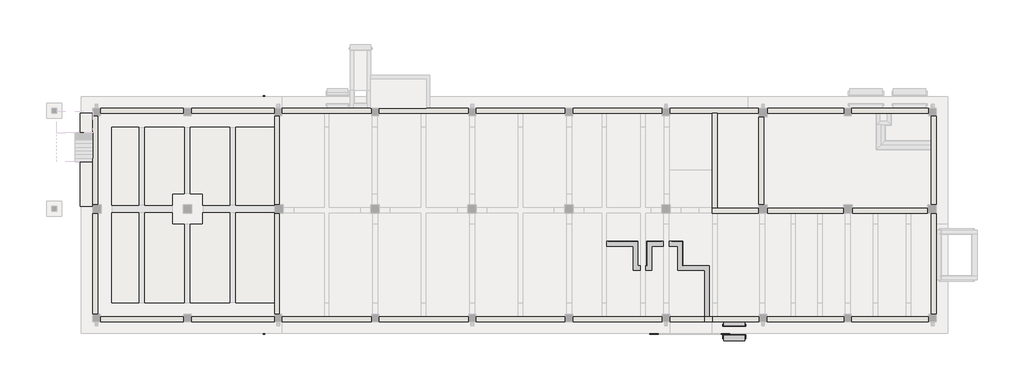
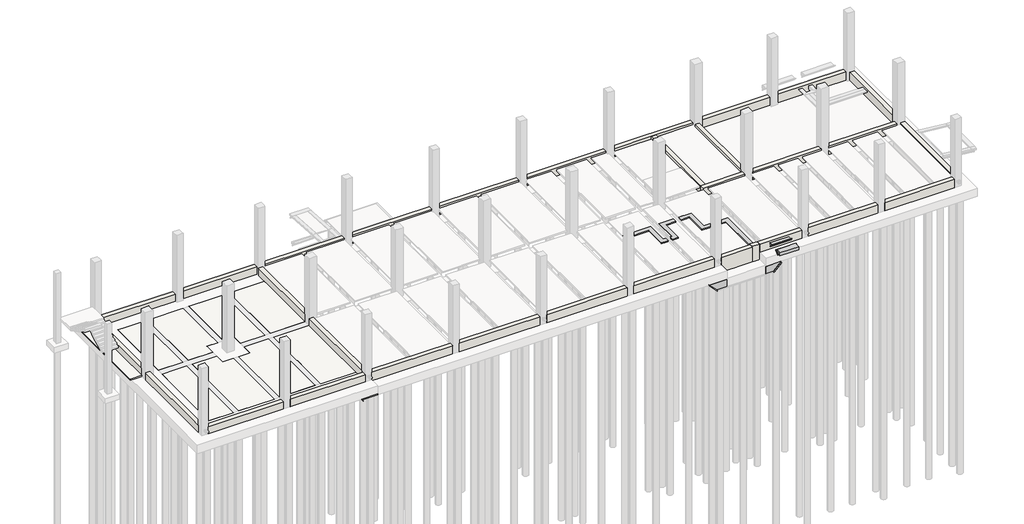
# One storey, part 1 of 7: 31 walls, 12 proxies, 4 slabs.
"""IFC4 building model written with IfcOpenShell, lengths in millimetres."""

from ifc_helpers import new_model, si_unit, frame, origin, place, context, project, spatial, polyline, outline, extrude, faceted_brep, element, save

model = new_model("IFC4")

# Units and contexts
model_context = context("Model", 3, world=origin())
ifc_project = project(units=[si_unit("LENGTHUNIT", "METRE", prefix="MILLI")], contexts=[model_context])

# Site, building, storey
site = spatial("IfcSite", under=ifc_project)
building = spatial("IfcBuilding", under=site)
storey = spatial("IfcBuildingStorey", under=building, Name="H.P.P", Elevation=4500.0)

# Proxies
placement = place(None, origin())
element("IfcBuildingElementProxy", 1, Name="H_SF_AR_S17_SOG Edge_1625x700", ObjectType="H_SF_AR_S17_SOG Edge_1625x700", at=placement, inside=storey, context=model_context, shape_type="SweptSolid", body=[
    extrude(outline(polyline([(2500.0, 47300.0), (3200.0, 47300.0), (3200.0, 45675.0), (2500.0, 46375.0), (2500.0, 47300.0)])), frame((0.0, -18250.0000001, 0.0), z_axis=(0.0, 1.0, 0.0), x_axis=(0.0, 0.0, 1.0)), (0.0, 0.0, 1.0), 2500.0),
])
element("IfcBuildingElementProxy", 2, Name="H_SF_AR_S17_SOG Edge_1400x700", ObjectType="H_SF_AR_S17_SOG Edge_1400x700", at=placement, inside=storey, context=model_context, shape_type="SweptSolid", body=[
    extrude(outline(polyline([(2500.0, 50825.0), (2500.0, 51525.0), (3200.0, 52225.0), (3200.0, 50825.0), (2500.0, 50825.0)])), frame((0.0, -18250.0000001, 0.0), z_axis=(0.0, 1.0, 0.0), x_axis=(0.0, 0.0, 1.0)), (0.0, 0.0, 1.0), 2500.0),
])
element("IfcBuildingElementProxy", 3, Name="H_SF_AR_S17_SOG Edge_1500x100", ObjectType="H_SF_AR_S17_SOG Edge_1500x100", at=placement, inside=storey, context=model_context, shape_type="SweptSolid", body=[
    extrude(outline(polyline([(3200.0, 15299.9999999), (3300.0, 15299.9999999), (3300.0, 13799.9999999), (3200.0, 13899.9999999), (3200.0, 15299.9999999)])), frame((0.0, -18250.0000001, 0.0), z_axis=(0.0, 1.0, 0.0), x_axis=(0.0, 0.0, 1.0)), (0.0, 0.0, 1.0), 2500.0),
    extrude(outline(polyline([(3200.0, 15299.9999999), (3300.0, 15299.9999999), (3300.0, 13799.9999999), (3200.0, 13899.9999999), (3200.0, 15299.9999999)])), frame((0.0, -1250.0000001, 0.0), z_axis=(0.0, 1.0, 0.0), x_axis=(0.0, 0.0, 1.0)), (0.0, 0.0, 1.0), 2500.0),
])
element("IfcBuildingElementProxy", 4, Name="H_SF_AR_S18_Lean_T50", ObjectType="H_SF_AR_S18_Lean_T50", at=placement, inside=storey, context=model_context, shape_type="SweptSolid", body=[
    extrude(outline(polyline([(3200.0, 52225.0), (2500.0, 51525.0), (2450.0, 51525.0), (2450.0, 51545.7106781), (3150.0, 52245.7106781), (3150.0, 52225.0), (3200.0, 52225.0)])), frame((0.0, -18350.0000001, 0.0), z_axis=(0.0, 1.0, 0.0), x_axis=(0.0, 0.0, 1.0)), (0.0, 0.0, 1.0), 2700.0),
])
element("IfcBuildingElementProxy", 5, Name="H_SF_AR_S18_Lean_T50", ObjectType="H_SF_AR_S18_Lean_T50", at=placement, inside=storey, context=model_context, shape_type="SweptSolid", body=[
    extrude(outline(polyline([(3200.0, 45675.0), (3150.0, 45675.0), (3150.0, 45654.2893219), (2450.0, 46354.2893219), (2450.0, 46375.0), (2500.0, 46375.0), (3200.0, 45675.0)])), frame((0.0, -18350.0000001, 0.0), z_axis=(0.0, 1.0, 0.0), x_axis=(0.0, 0.0, 1.0)), (0.0, 0.0, 1.0), 2700.0),
])
element("IfcBuildingElementProxy", 6, Name="H_SF_AR_S18_Lean_T50_100X100", ObjectType="H_SF_AR_S18_Lean_T50_100X100", at=placement, inside=storey, context=model_context, shape_type="SweptSolid", body=[
    extrude(outline(polyline([(3300.0, 13799.9999999), (3250.0, 13799.9999999), (3250.0, 13779.2893218), (3150.0, 13879.2893218), (3150.0, 13899.9999999), (3200.0, 13899.9999999), (3300.0, 13799.9999999)])), frame((0.0, -18350.0000001, 0.0), z_axis=(0.0, 1.0, 0.0), x_axis=(0.0, 0.0, 1.0)), (0.0, 0.0, 1.0), 2810.0),
    extrude(outline(polyline([(3300.0, 13799.9999999), (3250.0, 13799.9999999), (3250.0, 13779.2893218), (3150.0, 13879.2893218), (3150.0, 13899.9999999), (3200.0, 13899.9999999), (3300.0, 13799.9999999)])), frame((0.0, -1460.0000001, 0.0), z_axis=(0.0, 1.0, 0.0), x_axis=(0.0, 0.0, 1.0)), (0.0, 0.0, 1.0), 2810.0),
])
element("IfcBuildingElementProxy", 7, Name="H_SF_AR_B08_Stoop_T150_FrontEdge", ObjectType="H_SF_AR_B08_Stoop_T150_FrontEdge", at=placement, inside=storey, context=model_context, shape_type="SweptSolid", body=[
    extrude(outline(polyline([(-17312.0, 4450.0), (-17512.0, 4450.0), (-17662.0, 4600.0), (-17312.0, 4600.0), (-17312.0, 4450.0)])), frame((51775.0, 0.0, 0.0), z_axis=(1.0, 0.0, 0.0), x_axis=(0.0, 1.0, 0.0)), (0.0, 0.0, 1.0), 1700.0),
])
element("IfcBuildingElementProxy", 8, Name="H_SF_AR_B08_Stoop_T150_FrontEdge_500x300", ObjectType="H_SF_AR_B08_Stoop_T150_FrontEdge_500x300", at=placement, inside=storey, context=model_context, shape_type="Brep", body=[
    faceted_brep([(51775.0, -18899.9999926, 4300.0), (51775.0, -18899.9999926, 4600.0), (51775.0, -18599.9999926, 4600.0), (51775.0, -18399.9999926, 4600.0), (51775.0, -18699.9999926, 4300.0), (53475.0, -18899.9999926, 4300.0), (53475.0, -18699.9999926, 4300.0), (53475.0, -18399.9999926, 4600.0), (53475.0, -18599.9999926, 4600.0), (53475.0, -18899.9999926, 4600.0)], [[[0, 1, 2, 3, 4]], [[5, 6, 7, 8, 9]], [[1, 0, 5, 9]], [[3, 2, 1, 9, 8, 7]], [[4, 3, 7, 6]], [[0, 4, 6, 5]]]),
])
element("IfcBuildingElementProxy", 9, Name="H_SF_AR_S18_Lean_T50_300X300", ObjectType="H_SF_AR_S18_Lean_T50_300X300", at=placement, inside=storey, context=model_context, shape_type="SweptSolid", body=[
    extrude(outline(polyline([(-18699.9999926, 4250.0), (-18699.9999926, 4300.0), (-18399.9999926, 4600.0), (-18399.9999926, 4550.0), (-18379.2893145, 4550.0), (-18679.2893145, 4250.0), (-18699.9999926, 4250.0)])), frame((51675.0, 0.0, 0.0), z_axis=(1.0, 0.0, 0.0), x_axis=(0.0, 1.0, 0.0)), (0.0, 0.0, 1.0), 1900.0),
])
element("IfcBuildingElementProxy", 10, Name="H_SF_AR_S18_Lean_T50_150X150", ObjectType="H_SF_AR_S18_Lean_T50_150X150", at=placement, inside=storey, context=model_context, shape_type="SweptSolid", body=[
    extrude(outline(polyline([(-17512.0, 4450.0), (-17512.0, 4400.0), (-17532.7106781, 4400.0), (-17682.7106781, 4550.0), (-17662.0, 4550.0), (-17662.0, 4600.0), (-17512.0, 4450.0)])), frame((51675.0, 0.0, 0.0), z_axis=(1.0, 0.0, 0.0), x_axis=(0.0, 1.0, 0.0)), (0.0, 0.0, 1.0), 1900.0),
])
element("IfcBuildingElementProxy", 11, Name="H_SF_AR_S17_SOG Edge_450x150", ObjectType="H_SF_AR_S17_SOG Edge_450x150", at=placement, inside=storey, context=model_context, shape_type="Brep", body=[
    faceted_brep([(50175.0, -16900.0, 4550.0), (50475.0, -16900.0, 4550.0), (50575.0, -16900.0, 4650.0), (50175.0, -16900.0, 4650.0), (50175.0, -13075.0, 4550.0), (50175.0, -13075.0, 4650.0), (50475.0, -12775.0, 4550.0), (50575.0, -12675.0, 4650.0), (48375.0, -12675.0, 4650.0), (48375.0, -10675.0, 4650.0), (47250.0, -10675.0, 4650.0), (47250.0, -11075.0, 4650.0), (47975.0, -11075.0, 4650.0), (47975.0, -13075.0, 4650.0), (47975.0, -13075.0, 4550.0), (48275.0, -12775.0, 4550.0), (47975.0, -11075.0, 4550.0), (48275.0, -10775.0, 4550.0), (47250.0, -10775.0, 4550.0), (47250.0, -11075.0, 4550.0)], [[[0, 1, 2, 3]], [[4, 0, 3, 5]], [[1, 6, 7, 2]], [[4, 6, 1, 0]], [[3, 2, 7, 8, 9, 10, 11, 12, 13, 5]], [[4, 5, 13, 14]], [[7, 6, 15, 8]], [[6, 4, 14, 15]], [[14, 13, 12, 16]], [[8, 15, 17, 9]], [[15, 14, 16, 17]], [[18, 19, 11, 10]], [[16, 12, 11, 19]], [[9, 17, 18, 10]], [[17, 16, 19, 18]]]),
    faceted_brep([(46750.0, -11075.0, 4650.0), (46750.0, -10675.0, 4650.0), (45425.0, -10675.0, 4650.0), (45425.0, -12675.0, 4650.0), (45325.0, -12675.0, 4650.0), (45325.0, -13075.0, 4650.0), (45825.0, -13075.0, 4650.0), (45825.0, -11075.0, 4650.0), (46750.0, -11075.0, 4550.0), (46750.0, -10775.0, 4550.0), (45825.0, -11075.0, 4550.0), (45525.0, -10775.0, 4550.0), (45825.0, -13075.0, 4550.0), (45525.0, -12775.0, 4550.0), (45325.0, -12775.0, 4550.0), (45325.0, -13075.0, 4550.0)], [[[0, 1, 2, 3, 4, 5, 6, 7]], [[8, 9, 1, 0]], [[10, 8, 0, 7]], [[9, 11, 2, 1]], [[10, 11, 9, 8]], [[10, 7, 6, 12]], [[2, 11, 13, 3]], [[11, 10, 12, 13]], [[14, 15, 5, 4]], [[12, 6, 5, 15]], [[3, 13, 14, 4]], [[13, 12, 15, 14]]]),
    faceted_brep([(44875.0, -13075.0, 4650.0), (44875.0, -12675.0, 4650.0), (44675.0, -12675.0, 4650.0), (44675.0, -10675.0, 4650.0), (42125.0, -10675.0, 4650.0), (42125.0, -11075.0, 4650.0), (44275.0, -11075.0, 4650.0), (44275.0, -13075.0, 4650.0), (44875.0, -13075.0, 4550.0), (44875.0, -12775.0, 4550.0), (44275.0, -13075.0, 4550.0), (44575.0, -12775.0, 4550.0), (44275.0, -11075.0, 4550.0), (44575.0, -10775.0, 4550.0), (42125.0, -10775.0, 4550.0), (42125.0, -11075.0, 4550.0)], [[[0, 1, 2, 3, 4, 5, 6, 7]], [[8, 9, 1, 0]], [[10, 8, 0, 7]], [[9, 11, 2, 1]], [[10, 11, 9, 8]], [[10, 7, 6, 12]], [[2, 11, 13, 3]], [[11, 10, 12, 13]], [[14, 15, 5, 4]], [[12, 6, 5, 15]], [[3, 13, 14, 4]], [[13, 12, 15, 14]]]),
])
element("IfcBuildingElementProxy", 12, Name="H_SF_AR_S18_Lean_T50_100X100", ObjectType="H_SF_AR_S18_Lean_T50_100X100", at=placement, inside=storey, context=model_context, shape_type="Brep", body=[
    faceted_brep([(50575.0, -16790.0, 4540.0), (50475.0, -16790.0, 4440.0), (50475.0, -16790.0, 4390.0), (50495.7106781, -16790.0, 4390.0), (50595.7106781, -16790.0, 4490.0), (50575.0, -16790.0, 4490.0), (50575.0, -12675.0, 4490.0), (50575.0, -12675.0, 4540.0), (50595.7106781, -12654.2893219, 4490.0), (50495.7106781, -12754.2893219, 4390.0), (50475.0, -12775.0, 4390.0), (50475.0, -12775.0, 4440.0), (48375.0, -12675.0, 4540.0), (48275.0, -12775.0, 4440.0), (48275.0, -12775.0, 4390.0), (48295.7106781, -12754.2893219, 4390.0), (48395.7106781, -12654.2893219, 4490.0), (48375.0, -12675.0, 4490.0), (48375.0, -10675.0, 4540.0), (48275.0, -10775.0, 4440.0), (48275.0, -10775.0, 4390.0), (48295.7106781, -10754.2893219, 4390.0), (48395.7106781, -10654.2893219, 4490.0), (48375.0, -10675.0, 4490.0), (47360.0, -10675.0, 4540.0), (47360.0, -10675.0, 4490.0), (47360.0, -10654.2893219, 4490.0), (47360.0, -10754.2893219, 4390.0), (47360.0, -10775.0, 4390.0), (47360.0, -10775.0, 4440.0)], [[[0, 1, 2, 3, 4, 5]], [[0, 5, 6, 7]], [[5, 4, 8, 6]], [[4, 3, 9, 8]], [[3, 2, 10, 9]], [[2, 1, 11, 10]], [[1, 0, 7, 11]], [[11, 7, 12, 13]], [[10, 11, 13, 14]], [[9, 10, 14, 15]], [[8, 9, 15, 16]], [[6, 8, 16, 17]], [[7, 6, 17, 12]], [[13, 12, 18, 19]], [[14, 13, 19, 20]], [[15, 14, 20, 21]], [[16, 15, 21, 22]], [[17, 16, 22, 23]], [[12, 17, 23, 18]], [[24, 25, 26, 27, 28, 29]], [[19, 18, 24, 29]], [[20, 19, 29, 28]], [[21, 20, 28, 27]], [[22, 21, 27, 26]], [[23, 22, 26, 25]], [[18, 23, 25, 24]]]),
    faceted_brep([(46640.0, -10675.0, 4540.0), (46640.0, -10775.0, 4440.0), (46640.0, -10775.0, 4390.0), (46640.0, -10754.2893219, 4390.0), (46640.0, -10654.2893219, 4490.0), (46640.0, -10675.0, 4490.0), (45425.0, -10675.0, 4540.0), (45525.0, -10775.0, 4440.0), (45525.0, -10775.0, 4390.0), (45504.2893219, -10754.2893219, 4390.0), (45404.2893219, -10654.2893219, 4490.0), (45425.0, -10675.0, 4490.0), (45435.0, -10675.0, 4490.0), (45425.0, -12775.0, 4540.0), (45425.0, -12775.0, 4490.0), (45404.2893219, -12775.0, 4490.0), (45504.2893219, -12775.0, 4390.0), (45525.0, -12775.0, 4390.0), (45525.0, -12775.0, 4440.0)], [[[0, 1, 2, 3, 4, 5]], [[1, 0, 6, 7]], [[2, 1, 7, 8]], [[3, 2, 8, 9]], [[4, 3, 9, 10]], [[5, 4, 10, 11, 12]], [[0, 5, 12, 11, 6]], [[13, 14, 15, 16, 17, 18]], [[7, 6, 13, 18]], [[8, 7, 18, 17]], [[9, 8, 17, 16]], [[10, 9, 16, 15]], [[11, 10, 15, 14]], [[6, 11, 14, 13]]]),
    faceted_brep([(42235.0, -10675.0, 4540.0), (42235.0, -10675.0, 4490.0), (42235.0, -10654.2893219, 4490.0), (42235.0, -10754.2893219, 4390.0), (42235.0, -10775.0, 4390.0), (42235.0, -10775.0, 4440.0), (44575.0, -10775.0, 4440.0), (44675.0, -10675.0, 4540.0), (44575.0, -10775.0, 4390.0), (44595.7106781, -10754.2893219, 4390.0), (44695.7106781, -10654.2893219, 4490.0), (44675.0, -10675.0, 4490.0), (44575.0, -12775.0, 4440.0), (44675.0, -12675.0, 4540.0), (44575.0, -12775.0, 4390.0), (44595.7106781, -12754.2893219, 4390.0), (44695.7106781, -12654.2893219, 4490.0), (44675.0, -12675.0, 4490.0), (44765.0, -12675.0, 4540.0), (44765.0, -12775.0, 4440.0), (44765.0, -12775.0, 4390.0), (44765.0, -12754.2893219, 4390.0), (44765.0, -12654.2893219, 4490.0), (44765.0, -12675.0, 4490.0)], [[[0, 1, 2, 3, 4, 5]], [[6, 7, 0, 5]], [[8, 6, 5, 4]], [[9, 8, 4, 3]], [[10, 9, 3, 2]], [[11, 10, 2, 1]], [[7, 11, 1, 0]], [[12, 13, 7, 6]], [[14, 12, 6, 8]], [[15, 14, 8, 9]], [[16, 15, 9, 10]], [[17, 16, 10, 11]], [[13, 17, 11, 7]], [[18, 19, 20, 21, 22, 23]], [[19, 18, 13, 12]], [[20, 19, 12, 14]], [[21, 20, 14, 15]], [[22, 21, 15, 16]], [[23, 22, 16, 17]], [[18, 23, 17, 13]]]),
])

# Slabs
element("IfcSlab", 13, ObjectType="H_FL_AR_S17_RC Slab_T150_B1S1", at=placement, inside=storey, context=model_context, shape_type="Brep", body=[
    faceted_brep([(3500.0, -1250.0000001, 3950.0), (3500.0, -7700.0, 3950.0), (1250.0000002, -7700.0, 3950.0), (1250.0000002, -1250.0000001, 3950.0), (3500.0, -7700.0, 4100.0), (3500.0, -1250.0000001, 4100.0), (1250.0000002, -1250.0000001, 4100.0), (1250.0000002, -7700.0, 4100.0)], [[[0, 1, 2, 3]], [[4, 5, 6, 7]], [[1, 0, 5, 4]], [[2, 1, 4, 7]], [[3, 2, 7, 6]], [[0, 3, 6, 5]]]),
    faceted_brep([(1250.0000002, -8300.0, 3950.0), (3500.0, -8300.0, 3950.0), (3500.0, -15750.0000001, 3950.0), (1250.0000002, -15750.0000001, 3950.0), (3500.0, -8300.0, 4100.0), (1250.0000002, -8300.0, 4100.0), (1250.0000002, -15750.0000001, 4100.0), (3500.0, -15750.0000001, 4100.0)], [[[0, 1, 2, 3]], [[4, 5, 6, 7]], [[1, 0, 5, 4]], [[2, 1, 4, 7]], [[3, 2, 7, 6]], [[0, 3, 6, 5]]]),
    faceted_brep([(6250.0, -7700.0, 3950.0), (4000.0, -7700.0, 3950.0), (4000.0, -1250.0000001, 3950.0), (7250.0, -1250.0000001, 3950.0), (7250.0, -6750.0, 3950.0), (6250.0, -6750.0, 3950.0), (4000.0, -7700.0, 4100.0), (6250.0, -7700.0, 4100.0), (6250.0, -6750.0, 4100.0), (7250.0, -6750.0, 4100.0), (7250.0, -1250.0000001, 4100.0), (4000.0, -1250.0000001, 4100.0)], [[[0, 1, 2, 3, 4, 5]], [[6, 7, 8, 9, 10, 11]], [[1, 0, 7, 6]], [[2, 1, 6, 11]], [[3, 2, 11, 10]], [[4, 3, 10, 9]], [[5, 4, 9, 8]], [[0, 5, 8, 7]]]),
    faceted_brep([(6250.0, -8300.0, 3950.0), (6250.0, -9250.0, 3950.0), (7250.0, -9250.0, 3950.0), (7250.0, -15750.0000001, 3950.0), (4000.0, -15750.0000001, 3950.0), (4000.0, -8300.0, 3950.0), (6250.0, -9250.0, 4100.0), (6250.0, -8300.0, 4100.0), (4000.0, -8300.0, 4100.0), (4000.0, -15750.0000001, 4100.0), (7250.0, -15750.0000001, 4100.0), (7250.0, -9250.0, 4100.0)], [[[0, 1, 2, 3, 4, 5]], [[6, 7, 8, 9, 10, 11]], [[1, 0, 7, 6]], [[2, 1, 6, 11]], [[3, 2, 11, 10]], [[4, 3, 10, 9]], [[5, 4, 9, 8]], [[0, 5, 8, 7]]]),
    faceted_brep([(8750.0, -7700.0, 3950.0), (8750.0, -6750.0, 3950.0), (7750.0, -6750.0, 3950.0), (7750.0, -1250.0000001, 3950.0), (11000.0, -1250.0000001, 3950.0), (11000.0, -7700.0, 3950.0), (8750.0, -6750.0, 4100.0), (8750.0, -7700.0, 4100.0), (11000.0, -7700.0, 4100.0), (11000.0, -1250.0000001, 4100.0), (7750.0, -1250.0000001, 4100.0), (7750.0, -6750.0, 4100.0)], [[[0, 1, 2, 3, 4, 5]], [[6, 7, 8, 9, 10, 11]], [[1, 0, 7, 6]], [[2, 1, 6, 11]], [[3, 2, 11, 10]], [[4, 3, 10, 9]], [[5, 4, 9, 8]], [[0, 5, 8, 7]]]),
    faceted_brep([(8750.0, -8300.0, 3950.0), (11000.0, -8300.0, 3950.0), (11000.0, -15750.0000001, 3950.0), (7750.0, -15750.0000001, 3950.0), (7750.0, -9250.0, 3950.0), (8750.0, -9250.0, 3950.0), (11000.0, -8300.0, 4100.0), (8750.0, -8300.0, 4100.0), (8750.0, -9250.0, 4100.0), (7750.0, -9250.0, 4100.0), (7750.0, -15750.0000001, 4100.0), (11000.0, -15750.0000001, 4100.0)], [[[0, 1, 2, 3, 4, 5]], [[6, 7, 8, 9, 10, 11]], [[1, 0, 7, 6]], [[2, 1, 6, 11]], [[3, 2, 11, 10]], [[4, 3, 10, 9]], [[5, 4, 9, 8]], [[0, 5, 8, 7]]]),
    faceted_brep([(11500.0, -7699.9999999, 3950.0), (11500.0, -1250.0000001, 3950.0), (14700.0000001, -1250.0000001, 3950.0), (14700.0000001, -6750.0, 3950.0), (13800.0000001, -6750.0, 3950.0), (13800.0000001, -7699.9999999, 3950.0), (14700.0000001, -7699.9999999, 4100.0), (14700.0000001, -1250.0000001, 4100.0), (11500.0, -1250.0000001, 4100.0), (11500.0, -7699.9999999, 4100.0), (14700.0000001, -7699.9999999, 4000.0), (14700.0000001, -7650.0, 4000.0), (14700.0000001, -6750.0, 4000.0), (13800.0000001, -7699.9999999, 4000.0), (13800.0000001, -6750.0, 4000.0)], [[[0, 1, 2, 3, 4, 5]], [[6, 7, 8, 9]], [[7, 6, 10, 11, 12, 3, 2]], [[6, 9, 0, 5, 13, 10]], [[1, 0, 9, 8]], [[2, 1, 8, 7]], [[13, 14, 12, 11, 10]], [[12, 14, 4, 3]], [[14, 13, 5, 4]]]),
    faceted_brep([(14700.0, -15750.0000001, 3950.0), (11500.0, -15750.0000001, 3950.0), (11500.0, -8299.9999999, 3950.0), (13800.0000001, -8299.9999999, 3950.0), (13800.0000001, -9250.0, 3950.0), (14700.0, -9250.0, 3950.0), (14700.0, -15750.0000001, 4100.0), (14700.0, -8299.9999999, 4100.0), (11500.0, -8299.9999999, 4100.0), (11500.0, -15750.0000001, 4100.0), (14700.0, -9250.0, 4000.0), (14700.0, -8350.0, 4000.0), (14700.0, -8299.9999999, 4000.0), (13800.0000001, -8299.9999999, 4000.0), (13800.0000001, -9250.0, 4000.0)], [[[0, 1, 2, 3, 4, 5]], [[6, 7, 8, 9]], [[7, 6, 0, 5, 10, 11, 12]], [[1, 0, 6, 9]], [[2, 1, 9, 8]], [[8, 7, 12, 13, 3, 2]], [[10, 14, 13, 12, 11]], [[13, 14, 4, 3]], [[14, 10, 5, 4]]]),
])
element("IfcSlab", 14, ObjectType="H_FL_AR_B07_Ground Insulation_T110", at=placement, inside=storey, context=model_context, shape_type="SweptSolid", body=[
    extrude(outline(polyline([(3500.0, -1250.0000001), (3500.0, -7700.0), (1250.0000002, -7700.0), (1250.0000002, -1250.0000001), (3500.0, -1250.0000001)])), frame((0.0, 0.0, 3840.0), z_axis=(0.0, 0.0, 1.0), x_axis=(1.0, 0.0, 0.0)), (0.0, 0.0, 1.0), 110.0),
    extrude(outline(polyline([(3500.0, -8300.0), (3500.0, -15750.0000001), (1250.0000002, -15750.0000001), (1250.0000002, -8300.0), (3500.0, -8300.0)])), frame((0.0, 0.0, 3840.0), z_axis=(0.0, 0.0, 1.0), x_axis=(1.0, 0.0, 0.0)), (0.0, 0.0, 1.0), 110.0),
    extrude(outline(polyline([(6250.0, -8300.0), (6250.0, -9250.0), (7250.0, -9250.0), (7250.0, -15750.0000001), (4000.0, -15750.0000001), (4000.0, -8300.0), (6250.0, -8300.0)])), frame((0.0, 0.0, 3840.0), z_axis=(0.0, 0.0, 1.0), x_axis=(1.0, 0.0, 0.0)), (0.0, 0.0, 1.0), 110.0),
    extrude(outline(polyline([(6250.0, -7700.0), (4000.0, -7700.0), (4000.0, -1250.0000001), (7250.0, -1250.0000001), (7250.0, -6750.0), (6250.0, -6750.0), (6250.0, -7700.0)])), frame((0.0, 0.0, 3840.0), z_axis=(0.0, 0.0, 1.0), x_axis=(1.0, 0.0, 0.0)), (0.0, 0.0, 1.0), 110.0),
    extrude(outline(polyline([(8750.0, -8300.0), (11000.0, -8300.0), (11000.0, -15750.0000001), (7750.0, -15750.0000001), (7750.0, -9250.0), (8750.0, -9250.0), (8750.0, -8300.0)])), frame((0.0, 0.0, 3840.0), z_axis=(0.0, 0.0, 1.0), x_axis=(1.0, 0.0, 0.0)), (0.0, 0.0, 1.0), 110.0),
    extrude(outline(polyline([(8750.0, -7700.0), (8750.0, -6750.0), (7750.0, -6750.0), (7750.0, -1250.0000001), (11000.0, -1250.0000001), (11000.0, -7700.0), (8750.0, -7700.0)])), frame((0.0, 0.0, 3840.0), z_axis=(0.0, 0.0, 1.0), x_axis=(1.0, 0.0, 0.0)), (0.0, 0.0, 1.0), 110.0),
    extrude(outline(polyline([(13800.0000001, -8300.0), (13800.0000001, -9250.0), (14700.0, -9250.0), (14700.0, -15750.0000001), (11500.0, -15750.0000001), (11500.0, -8300.0), (13800.0000001, -8300.0)])), frame((0.0, 0.0, 3840.0), z_axis=(0.0, 0.0, 1.0), x_axis=(1.0, 0.0, 0.0)), (0.0, 0.0, 1.0), 110.0),
    extrude(outline(polyline([(13800.0000001, -7700.0), (11500.0, -7700.0), (11500.0, -1250.0000001), (14700.0, -1250.0000001), (14700.0, -6750.0), (13800.0000001, -6750.0), (13800.0000001, -7700.0)])), frame((0.0, 0.0, 3840.0), z_axis=(0.0, 0.0, 1.0), x_axis=(1.0, 0.0, 0.0)), (0.0, 0.0, 1.0), 110.0),
])
element("IfcSlab", 15, ObjectType="H_FL_AR_B07_Ground Insulation_T110", at=placement, inside=storey, context=model_context, shape_type="Brep", body=[
    faceted_brep([(50575.0, -16900.0, 4540.0), (50575.0, -16900.0, 4650.0), (50475.0, -16900.0, 4550.0), (50475.0, -16900.0, 4440.0), (50475.0, -12775.0, 4550.0), (50475.0, -12775.0, 4440.0), (48275.0, -12775.0, 4550.0), (48275.0, -12775.0, 4440.0), (48375.0, -12675.0, 4540.0), (48375.0, -12675.0, 4650.0), (50575.0, -12675.0, 4650.0), (50575.0, -12675.0, 4540.0), (47459.9999996, -10675.0, 4540.0), (47459.9999996, -10675.0, 4650.0), (48375.0, -10675.0, 4650.0), (48375.0, -10675.0, 4540.0), (48275.0, -10775.0, 4440.0), (48275.0, -10775.0, 4550.0), (47459.9999996, -10775.0, 4550.0), (47459.9999996, -10775.0, 4440.0)], [[[0, 1, 2, 3]], [[3, 2, 4, 5]], [[5, 4, 6, 7]], [[8, 9, 10, 11]], [[11, 10, 1, 0]], [[10, 4, 2, 1]], [[11, 0, 3, 5]], [[12, 13, 14, 15]], [[16, 17, 18, 19]], [[19, 18, 13, 12]], [[7, 6, 17, 16]], [[15, 14, 9, 8]], [[18, 17, 14, 13]], [[10, 9, 6, 4]], [[19, 12, 15, 16]], [[11, 5, 7, 8]], [[9, 14, 17, 6]], [[8, 7, 16, 15]]]),
    faceted_brep([(46640.0, -10675.0, 4540.0), (46640.0, -10675.0, 4650.0), (46640.0, -10775.0, 4550.0), (46640.0, -10775.0, 4440.0), (45525.0, -10775.0, 4550.0), (45525.0, -10775.0, 4440.0), (45525.0, -12775.0, 4550.0), (45525.0, -12775.0, 4440.0), (45325.0, -12775.0, 4550.0), (45325.0, -12775.0, 4440.0), (45425.0, -12675.0, 4540.0), (45425.0, -12675.0, 4650.0), (45425.0, -10675.0, 4650.0), (45425.0, -10675.0, 4540.0), (45325.0, -12675.0, 4650.0), (45325.0, -12675.0, 4540.0)], [[[0, 1, 2, 3]], [[3, 2, 4, 5]], [[5, 4, 6, 7]], [[7, 6, 8, 9]], [[10, 11, 12, 13]], [[13, 12, 1, 0]], [[12, 4, 2, 1]], [[13, 0, 3, 5]], [[9, 8, 14, 15]], [[15, 14, 11, 10]], [[6, 11, 14, 8]], [[12, 11, 6, 4]], [[7, 9, 15, 10]], [[13, 5, 7, 10]]]),
    faceted_brep([(42235.0, -10675.0, 4540.0), (42235.0, -10675.0, 4650.0), (44675.0, -10675.0, 4650.0), (44675.0, -10675.0, 4540.0), (44675.0, -12675.0, 4650.0), (44675.0, -12675.0, 4540.0), (44875.0, -12775.0, 4440.0), (44875.0, -12775.0, 4550.0), (44575.0, -12775.0, 4550.0), (44575.0, -12775.0, 4440.0), (44575.0, -10775.0, 4550.0), (44575.0, -10775.0, 4440.0), (42235.0, -10775.0, 4550.0), (42235.0, -10775.0, 4440.0), (44875.0, -12675.0, 4650.0), (44875.0, -12675.0, 4540.0)], [[[0, 1, 2, 3]], [[3, 2, 4, 5]], [[6, 7, 8, 9]], [[9, 8, 10, 11]], [[11, 10, 12, 13]], [[13, 12, 1, 0]], [[12, 10, 2, 1]], [[13, 0, 3, 11]], [[10, 8, 4, 2]], [[11, 3, 5, 9]], [[5, 4, 14, 15]], [[15, 14, 7, 6]], [[8, 7, 14, 4]], [[9, 5, 15, 6]]]),
])
element("IfcSlab", 16, ObjectType="H_FL_AR_B07_Ground Insulation_T110", at=placement, inside=storey, context=model_context, shape_type="SweptSolid", body=[
    extrude(outline(polyline([(-300.0, -100.0), (-300.0, -7800.0), (-1360.0, -7800.0), (-1360.0, -100.0), (-300.0, -100.0)])), frame((0.0, 0.0, 4100.0), z_axis=(0.0, 0.0, 1.0), x_axis=(1.0, 0.0, 0.0)), (0.0, 0.0, 1.0), 110.0),
])

# Walls
element("IfcWall", 17, ObjectType="H_WA_AR_B02_Ext Wall RC-UG_T400_W1A", at=placement, inside=storey, context=model_context, shape_type="Brep", body=[
    faceted_brep([(300.0, -17300.0, 4100.0), (7200.0, -17300.0, 4100.0), (7200.0, -17300.0, 4800.0), (300.0, -17300.0, 4800.0), (300.0, -16900.0, 4100.0), (300.0, -16900.0, 4800.0), (7200.0, -16900.0, 4800.0), (7200.0, -16900.0, 4100.0), (7200.0, -17050.0, 4800.0), (300.0, -17050.0, 4800.0)], [[[0, 1, 2, 3]], [[4, 5, 6, 7]], [[1, 0, 4, 7]], [[2, 1, 7, 6, 8]], [[3, 2, 8, 6, 5, 9]], [[0, 3, 9, 5, 4]]]),
])
element("IfcWall", 18, ObjectType="H_WA_AR_B02_Ext Wall RC-UG_T400_W1A", at=placement, inside=storey, context=model_context, shape_type="Brep", body=[
    faceted_brep([(7800.0, -17300.0, 4100.0), (14700.0, -17300.0, 4100.0), (14700.0, -17300.0, 4800.0), (7800.0, -17300.0, 4800.0), (7800.0, -16900.0, 4100.0), (7800.0, -16900.0, 4800.0), (14700.0, -16900.0, 4800.0), (14700.0, -16900.0, 4100.0), (14700.0, -17050.0, 4800.0), (7800.0, -17050.0, 4800.0)], [[[0, 1, 2, 3]], [[4, 5, 6, 7]], [[1, 0, 4, 7]], [[2, 1, 7, 6, 8]], [[3, 2, 8, 6, 5, 9]], [[0, 3, 9, 5, 4]]]),
])
element("IfcWall", 19, ObjectType="H_WA_AR_B02_Ext Wall RC-UG_T400_W1A", at=placement, inside=storey, context=model_context, shape_type="Brep", body=[
    faceted_brep([(15299.9999999, -17300.0, 4000.0), (22700.0, -17300.0, 4000.0), (22700.0, -17300.0, 4800.0), (15299.9999999, -17300.0, 4800.0), (15299.9999999, -17300.0, 4100.0), (15299.9999999, -16900.0, 4000.0), (15299.9999999, -16900.0, 4800.0), (22700.0, -16900.0, 4800.0), (22700.0, -16900.0, 4000.0), (22700.0, -17050.0, 4800.0), (15299.9999999, -17050.0, 4800.0)], [[[0, 1, 2, 3, 4]], [[5, 6, 7, 8]], [[1, 0, 5, 8]], [[2, 1, 8, 7, 9]], [[3, 2, 9, 7, 6, 10]], [[0, 4, 3, 10, 6, 5]]]),
])
element("IfcWall", 20, ObjectType="H_WA_AR_B02_Ext Wall RC-UG_T400_W1A", at=placement, inside=storey, context=model_context, shape_type="Brep", body=[
    faceted_brep([(23300.0, -17300.0, 4000.0), (30700.0, -17300.0, 4000.0), (30700.0, -17300.0, 4800.0), (23300.0, -17300.0, 4800.0), (23300.0, -16900.0, 4000.0), (23300.0, -16900.0, 4800.0), (30700.0, -16900.0, 4800.0), (30700.0, -16900.0, 4000.0), (30700.0, -17050.0, 4800.0), (23300.0, -17050.0, 4800.0)], [[[0, 1, 2, 3]], [[4, 5, 6, 7]], [[1, 0, 4, 7]], [[2, 1, 7, 6, 8]], [[3, 2, 8, 6, 5, 9]], [[0, 3, 9, 5, 4]]]),
])
element("IfcWall", 21, ObjectType="H_WA_AR_B02_Ext Wall RC-UG_T400_W1A", at=placement, inside=storey, context=model_context, shape_type="Brep", body=[
    faceted_brep([(31300.0, -17300.0, 4000.0), (38700.0, -17300.0, 4000.0), (38700.0, -17300.0, 4800.0), (31300.0, -17300.0, 4800.0), (31300.0, -16900.0, 4000.0), (31300.0, -16900.0, 4800.0), (38700.0, -16900.0, 4800.0), (38700.0, -16900.0, 4000.0), (38700.0, -17050.0, 4800.0), (31300.0, -17050.0, 4800.0)], [[[0, 1, 2, 3]], [[4, 5, 6, 7]], [[1, 0, 4, 7]], [[2, 1, 7, 6, 8]], [[3, 2, 8, 6, 5, 9]], [[0, 3, 9, 5, 4]]]),
])
element("IfcWall", 22, ObjectType="H_WA_AR_B02_Ext Wall RC-UG_T400_W1A", at=placement, inside=storey, context=model_context, shape_type="Brep", body=[
    faceted_brep([(39300.0, -17300.0, 4000.0), (46700.0, -17300.0, 4000.0), (46700.0, -17300.0, 4800.0), (39300.0, -17300.0, 4800.0), (39300.0, -16900.0, 4000.0), (39300.0, -16900.0, 4800.0), (46700.0, -16900.0, 4800.0), (46700.0, -16900.0, 4000.0), (46700.0, -17050.0, 4800.0), (39300.0, -17050.0, 4800.0)], [[[0, 1, 2, 3]], [[4, 5, 6, 7]], [[1, 0, 4, 7]], [[2, 1, 7, 6, 8]], [[3, 2, 8, 6, 5, 9]], [[0, 3, 9, 5, 4]]]),
])
element("IfcWall", 23, ObjectType="H_WA_AR_B02_Ext Wall RC-UG_T400_W1A", at=placement, inside=storey, context=model_context, shape_type="Brep", body=[
    faceted_brep([(47300.0, -17300.0, 3300.0), (50175.0, -17300.0, 3300.0), (50175.0, -17300.0, 4700.0), (47300.0, -17300.0, 4700.0), (47300.0, -17300.0, 4000.0), (47300.0, -16900.0, 3300.0), (47300.0, -16900.0, 4700.0), (50175.0, -16900.0, 4700.0), (50175.0, -16900.0, 3300.0), (50175.0, -17050.0, 4700.0), (47300.0, -17050.0, 4700.0)], [[[0, 1, 2, 3, 4]], [[5, 6, 7, 8]], [[1, 0, 5, 8]], [[2, 1, 8, 7, 9]], [[3, 2, 9, 7, 6, 10]], [[0, 4, 3, 10, 6, 5]]]),
])
element("IfcWall", 24, ObjectType="H_WA_AR_B02_Ext Wall RC-UG_T400_W1A", at=placement, inside=storey, context=model_context, shape_type="Brep", body=[
    faceted_brep([(50175.0, -17300.0, 3300.0), (50825.0, -17300.0, 3300.0), (50825.0, -17300.0, 4000.0), (50825.0, -17300.0, 4800.0), (50175.0, -17300.0, 4800.0), (50175.0, -17300.0, 4700.0), (50175.0, -16900.0, 3300.0), (50175.0, -16900.0, 4700.0), (50175.0, -16900.0, 4800.0), (50825.0, -16900.0, 4800.0), (50825.0, -16900.0, 4000.0), (50825.0, -16900.0, 3300.0), (50175.0, -17050.0, 4800.0)], [[[0, 1, 2, 3, 4, 5]], [[6, 7, 8, 9, 10, 11]], [[1, 0, 6, 11]], [[3, 2, 1, 11, 10, 9]], [[4, 3, 9, 8, 12]], [[0, 5, 4, 12, 8, 7, 6]]]),
])
element("IfcWall", 25, ObjectType="H_WA_AR_B02_Ext Wall RC-UG_T400_W1A", at=placement, inside=storey, context=model_context, shape_type="Brep", body=[
    faceted_brep([(50825.0, -17300.0, 4000.0), (54700.0, -17300.0, 4000.0), (54700.0, -17300.0, 4800.0), (53175.0, -17300.0, 4800.0), (52075.0, -17300.0, 4800.0), (50825.0, -17300.0, 4800.0), (50825.0, -16900.0, 4000.0), (50825.0, -16900.0, 4800.0), (54700.0, -16900.0, 4800.0), (54700.0, -16900.0, 4000.0), (54700.0, -17050.0, 4800.0)], [[[0, 1, 2, 3, 4, 5]], [[6, 7, 8, 9]], [[1, 0, 6, 9]], [[2, 1, 9, 8, 10]], [[5, 4, 3, 2, 10, 8, 7]], [[0, 5, 7, 6]]]),
])
element("IfcWall", 26, ObjectType="H_WA_AR_B02_Ext Wall RC-UG_T400_W1A", at=placement, inside=storey, context=model_context, shape_type="Brep", body=[
    faceted_brep([(55300.0, -17300.0, 4000.0), (61700.0, -17300.0, 4000.0), (61700.0, -17300.0, 4800.0), (55300.0, -17300.0, 4800.0), (55300.0, -16900.0, 4000.0), (55300.0, -16900.0, 4800.0), (61700.0, -16900.0, 4800.0), (61700.0, -16900.0, 4000.0), (61700.0, -17050.0, 4800.0), (55300.0, -17050.0, 4800.0)], [[[0, 1, 2, 3]], [[4, 5, 6, 7]], [[1, 0, 4, 7]], [[2, 1, 7, 6, 8]], [[3, 2, 8, 6, 5, 9]], [[0, 3, 9, 5, 4]]]),
])
element("IfcWall", 27, ObjectType="H_WA_AR_B02_Ext Wall RC-UG_T400_W1A", at=placement, inside=storey, context=model_context, shape_type="Brep", body=[
    faceted_brep([(62300.0, -17300.0, 4000.0), (68700.0, -17300.0, 4000.0), (68700.0, -17300.0, 4800.0), (62300.0, -17300.0, 4800.0), (62300.0, -16900.0, 4000.0), (62300.0, -16900.0, 4800.0), (68700.0, -16900.0, 4800.0), (68700.0, -16900.0, 4000.0), (68700.0, -17050.0, 4800.0), (62300.0, -17050.0, 4800.0)], [[[0, 1, 2, 3]], [[4, 5, 6, 7]], [[1, 0, 4, 7]], [[2, 1, 7, 6, 8]], [[3, 2, 8, 6, 5, 9]], [[0, 3, 9, 5, 4]]]),
])
element("IfcWall", 28, ObjectType="H_WA_AR_B02_Ext Wall RC-UG_T400_W1A", at=placement, inside=storey, context=model_context, shape_type="Brep", body=[
    faceted_brep([(69300.0, -16700.0, 4000.0), (69300.0, -8350.0, 4000.0), (69300.0, -8350.0, 4800.0), (69300.0, -10250.0, 4800.0), (69300.0, -13350.0, 4800.0), (69300.0, -16700.0, 4800.0), (68900.0, -16700.0, 4000.0), (68900.0, -16700.0, 4800.0), (68900.0, -8350.0, 4800.0), (68900.0, -8350.0, 4000.0), (69050.0, -8350.0, 4800.0), (69050.0, -16700.0, 4800.0)], [[[0, 1, 2, 3, 4, 5]], [[6, 7, 8, 9]], [[1, 0, 6, 9]], [[2, 1, 9, 8, 10]], [[5, 4, 3, 2, 10, 8, 7, 11]], [[0, 5, 11, 7, 6]]]),
])
element("IfcWall", 29, ObjectType="H_WA_AR_B02_Ext Wall RC-UG_T400_W1A", at=placement, inside=storey, context=model_context, shape_type="Brep", body=[
    faceted_brep([(69300.0, -7650.0, 4000.0), (69300.0, -300.0, 4000.0), (69300.0, -300.0, 4800.0), (69300.0, -7650.0, 4800.0), (68900.0, -7650.0, 4000.0), (68900.0, -7650.0, 4800.0), (68900.0, -300.0, 4800.0), (68900.0, -300.0, 4000.0), (69050.0, -300.0, 4800.0), (69050.0, -7650.0, 4800.0)], [[[0, 1, 2, 3]], [[4, 5, 6, 7]], [[1, 0, 4, 7]], [[2, 1, 7, 6, 8]], [[3, 2, 8, 6, 5, 9]], [[0, 3, 9, 5, 4]]]),
])
element("IfcWall", 30, ObjectType="H_WA_AR_B02_Ext Wall RC-UG_T400_W1A", at=placement, inside=storey, context=model_context, shape_type="Brep", body=[
    faceted_brep([(68700.0, 300.0, 4000.0), (62300.0, 300.0, 4000.0), (62300.0, 300.0, 4800.0), (62450.0, 300.0, 4800.0), (64550.0, 300.0, 4800.0), (66050.0, 300.0, 4800.0), (68150.0, 300.0, 4800.0), (68700.0, 300.0, 4800.0), (68700.0, -100.0, 4000.0), (68700.0, -100.0, 4800.0), (62300.0, -100.0, 4800.0), (62300.0, -100.0, 4000.0), (62300.0, 50.0, 4800.0), (68700.0, 50.0, 4800.0)], [[[0, 1, 2, 3, 4, 5, 6, 7]], [[8, 9, 10, 11]], [[1, 0, 8, 11]], [[2, 1, 11, 10, 12]], [[7, 6, 5, 4, 3, 2, 12, 10, 9, 13]], [[0, 7, 13, 9, 8]]]),
])
element("IfcWall", 31, ObjectType="H_WA_AR_B02_Ext Wall RC-UG_T400_W1A", at=placement, inside=storey, context=model_context, shape_type="Brep", body=[
    faceted_brep([(61700.0, 300.0, 4000.0), (55350.0, 300.0, 4000.0), (55350.0, 300.0, 4800.0), (61700.0, 300.0, 4800.0), (61700.0, -100.0, 4000.0), (61700.0, -100.0, 4800.0), (55350.0, -100.0, 4800.0), (55350.0, -100.0, 4000.0), (55350.0, 50.0, 4800.0), (61700.0, 50.0, 4800.0)], [[[0, 1, 2, 3]], [[4, 5, 6, 7]], [[1, 0, 4, 7]], [[2, 1, 7, 6, 8]], [[3, 2, 8, 6, 5, 9]], [[0, 3, 9, 5, 4]]]),
])
element("IfcWall", 32, ObjectType="H_WA_AR_B02_Ext Wall RC-UG_T400_W1A", at=placement, inside=storey, context=model_context, shape_type="Brep", body=[
    faceted_brep([(54650.0, 300.0, 4000.0), (47300.0, 300.0, 4000.0), (47300.0, 300.0, 4800.0), (54650.0, 300.0, 4800.0), (54650.0, -100.0, 4000.0), (54650.0, -100.0, 4800.0), (51225.0, -100.0, 4800.0), (50825.0, -100.0, 4800.0), (47300.0, -100.0, 4800.0), (47300.0, -100.0, 4000.0), (50825.0, -100.0, 4000.0), (51225.0, -100.0, 4000.0), (47300.0, 50.0, 4800.0), (54650.0, 50.0, 4800.0)], [[[0, 1, 2, 3]], [[4, 5, 6, 7, 8, 9, 10, 11]], [[1, 0, 4, 11, 10, 9]], [[2, 1, 9, 8, 12]], [[3, 2, 12, 8, 7, 6, 5, 13]], [[0, 3, 13, 5, 4]]]),
])
element("IfcWall", 33, ObjectType="H_WA_AR_B02_Ext Wall RC-UG_T400_W1A", at=placement, inside=storey, context=model_context, shape_type="Brep", body=[
    faceted_brep([(46700.0, 300.0, 4000.0), (39300.0, 300.0, 4000.0), (39300.0, 300.0, 4800.0), (46700.0, 300.0, 4800.0), (46700.0, -100.0, 4000.0), (46700.0, -100.0, 4800.0), (39300.0, -100.0, 4800.0), (39300.0, -100.0, 4000.0), (39300.0, 50.0, 4800.0), (46700.0, 50.0, 4800.0)], [[[0, 1, 2, 3]], [[4, 5, 6, 7]], [[1, 0, 4, 7]], [[2, 1, 7, 6, 8]], [[3, 2, 8, 6, 5, 9]], [[0, 3, 9, 5, 4]]]),
])
element("IfcWall", 34, ObjectType="H_WA_AR_B02_Ext Wall RC-UG_T400_W1A", at=placement, inside=storey, context=model_context, shape_type="Brep", body=[
    faceted_brep([(38700.0, 300.0, 4000.0), (31300.0, 300.0, 4000.0), (31300.0, 300.0, 4800.0), (38700.0, 300.0, 4800.0), (38700.0, -100.0, 4000.0), (38700.0, -100.0, 4800.0), (31300.0, -100.0, 4800.0), (31300.0, -100.0, 4000.0), (31300.0, 50.0, 4800.0), (38700.0, 50.0, 4800.0)], [[[0, 1, 2, 3]], [[4, 5, 6, 7]], [[1, 0, 4, 7]], [[2, 1, 7, 6, 8]], [[3, 2, 8, 6, 5, 9]], [[0, 3, 9, 5, 4]]]),
])
element("IfcWall", 35, ObjectType="H_WA_AR_B02_Ext Wall RC-UG_T400_W1A", at=placement, inside=storey, context=model_context, shape_type="Brep", body=[
    faceted_brep([(30700.0, 300.0, 4000.0), (23300.0, 300.0, 4000.0), (23300.0, 300.0, 4800.0), (30700.0, 300.0, 4800.0), (30700.0, -100.0, 4000.0), (30700.0, -100.0, 4800.0), (23300.0, -100.0, 4800.0), (23300.0, -100.0, 4000.0), (23300.0, 50.0, 4800.0), (30700.0, 50.0, 4800.0)], [[[0, 1, 2, 3]], [[4, 5, 6, 7]], [[1, 0, 4, 7]], [[2, 1, 7, 6, 8]], [[3, 2, 8, 6, 5, 9]], [[0, 3, 9, 5, 4]]]),
])
element("IfcWall", 36, ObjectType="H_WA_AR_B02_Ext Wall RC-UG_T400_W1A", at=placement, inside=storey, context=model_context, shape_type="Brep", body=[
    faceted_brep([(22700.0, 300.0, 4000.0), (15300.0, 300.0, 4000.0), (15300.0, 300.0, 4100.0), (15300.0, 300.0, 4800.0), (22690.0, 300.0, 4800.0), (22700.0, 300.0, 4800.0), (22700.0, -100.0, 4000.0), (22700.0, -100.0, 4800.0), (15300.0, -100.0, 4800.0), (15300.0, -100.0, 4000.0), (15300.0, 50.0, 4800.0)], [[[0, 1, 2, 3, 4, 5]], [[6, 7, 8, 9]], [[1, 0, 6, 9]], [[3, 2, 1, 9, 8, 10]], [[5, 4, 3, 10, 8, 7]], [[0, 5, 7, 6]]]),
])
element("IfcWall", 37, ObjectType="H_WA_AR_B02_Ext Wall RC-UG_T400_W1A", at=placement, inside=storey, context=model_context, shape_type="Brep", body=[
    faceted_brep([(14700.0, 300.0, 4100.0), (7800.0, 300.0, 4100.0), (7800.0, 300.0, 4800.0), (14700.0, 300.0, 4800.0), (14700.0, -100.0, 4100.0), (14700.0, -100.0, 4800.0), (7800.0, -100.0, 4800.0), (7800.0, -100.0, 4100.0), (7800.0, 50.0, 4800.0), (14700.0, 50.0, 4800.0)], [[[0, 1, 2, 3]], [[4, 5, 6, 7]], [[1, 0, 4, 7]], [[2, 1, 7, 6, 8]], [[3, 2, 8, 6, 5, 9]], [[0, 3, 9, 5, 4]]]),
])
element("IfcWall", 38, ObjectType="H_WA_AR_B02_Ext Wall RC-UG_T400_W1A", at=placement, inside=storey, context=model_context, shape_type="Brep", body=[
    faceted_brep([(7200.0, 300.0, 4100.0), (300.0, 300.0, 4100.0), (300.0, 300.0, 4800.0), (7200.0, 300.0, 4800.0), (7200.0, -100.0, 4100.0), (7200.0, -100.0, 4800.0), (300.0, -100.0, 4800.0), (300.0, -100.0, 4100.0), (300.0, 50.0, 4800.0), (7200.0, 50.0, 4800.0)], [[[0, 1, 2, 3]], [[4, 5, 6, 7]], [[1, 0, 4, 7]], [[2, 1, 7, 6, 8]], [[3, 2, 8, 6, 5, 9]], [[0, 3, 9, 5, 4]]]),
])
element("IfcWall", 39, ObjectType="H_WA_AR_B02_Ext Wall RC-UG_T400_W1A", at=placement, inside=storey, context=model_context, shape_type="Brep", body=[
    faceted_brep([(-300.0, -300.0, 4100.0), (-300.0, -7650.0, 4100.0), (-300.0, -7650.0, 4800.0), (-300.0, -300.0, 4800.0), (100.0, -300.0, 4100.0), (100.0, -300.0, 4800.0), (100.0, -7650.0, 4800.0), (100.0, -7650.0, 4100.0), (-50.0, -7650.0, 4800.0), (-50.0, -300.0, 4800.0)], [[[0, 1, 2, 3]], [[4, 5, 6, 7]], [[1, 0, 4, 7]], [[2, 1, 7, 6, 8]], [[3, 2, 8, 6, 5, 9]], [[0, 3, 9, 5, 4]]]),
])
element("IfcWall", 40, ObjectType="H_WA_AR_B02_Ext Wall RC-UG_T400_W1A", at=placement, inside=storey, context=model_context, shape_type="Brep", body=[
    faceted_brep([(-300.0, -8350.0, 4100.0), (-300.0, -16700.0, 4100.0), (-300.0, -16700.0, 4800.0), (-300.0, -8350.0, 4800.0), (100.0, -8350.0, 4100.0), (100.0, -8350.0, 4800.0), (100.0, -16700.0, 4800.0), (100.0, -16700.0, 4100.0), (-50.0, -16700.0, 4800.0), (-50.0, -8350.0, 4800.0)], [[[0, 1, 2, 3]], [[4, 5, 6, 7]], [[1, 0, 4, 7]], [[2, 1, 7, 6, 8]], [[3, 2, 8, 6, 5, 9]], [[0, 3, 9, 5, 4]]]),
])
element("IfcWall", 41, ObjectType="H_WA_AR_B02_Ext Wall RC-UG_T400_W2A", at=placement, inside=storey, context=model_context, shape_type="Brep", body=[
    faceted_brep([(14700.0, -300.0, 4100.0), (14700.0, -7650.0, 4100.0), (14700.0, -7650.0, 4800.0), (14700.0, -300.0, 4800.0), (15100.0, -300.0, 4100.0), (15100.0, -300.0, 4800.0), (15100.0, -7650.0, 4800.0), (15100.0, -7650.0, 4100.0), (14794.7873816, -7650.0, 4100.0)], [[[0, 1, 2, 3]], [[4, 5, 6, 7]], [[1, 0, 4, 7, 8]], [[2, 1, 8, 7, 6]], [[3, 2, 6, 5]], [[0, 3, 5, 4]]]),
])
element("IfcWall", 42, ObjectType="H_WA_AR_B02_Ext Wall RC-UG_T400_W2A", at=placement, inside=storey, context=model_context, shape_type="Brep", body=[
    faceted_brep([(14700.0, -8350.0, 4100.0), (14700.0, -16700.0, 4100.0), (14700.0, -16700.0, 4800.0), (14700.0, -8350.0, 4800.0), (15100.0, -8350.0, 4100.0), (15100.0, -8350.0, 4800.0), (15100.0, -16700.0, 4800.0), (15100.0, -16700.0, 4100.0), (14795.4630603, -8350.0, 4100.0)], [[[0, 1, 2, 3]], [[4, 5, 6, 7]], [[1, 0, 8, 4, 7]], [[2, 1, 7, 6]], [[3, 2, 6, 5]], [[0, 3, 5, 4, 8]]]),
])
element("IfcWall", 43, ObjectType="H_WA_AR_B02_Ext Wall RC-UG_T400_W2A", at=placement, inside=storey, context=model_context, shape_type="SweptSolid", body=[
    extrude(outline(polyline([(50825.0, -7950.0), (50825.0, -100.0), (51225.0, -100.0), (51225.0, -7950.0), (50825.0, -7950.0)])), frame((0.0, 0.0, 4000.0), z_axis=(0.0, 0.0, 1.0), x_axis=(1.0, 0.0, 0.0)), (0.0, 0.0, 1.0), 800.0),
])
element("IfcWall", 44, ObjectType="H_WA_AR_B02_Ext Wall RC-UG_T400_W2A", at=placement, inside=storey, context=model_context, shape_type="Brep", body=[
    faceted_brep([(54650.0, -7950.0, 4000.0), (51225.0, -7950.0, 4000.0), (50825.0, -7950.0, 4000.0), (50825.0, -7950.0, 4800.0), (51225.0, -7950.0, 4800.0), (54650.0, -7950.0, 4800.0), (54650.0, -8350.0, 4000.0), (54650.0, -8350.0, 4800.0), (50825.0, -8350.0, 4800.0), (50825.0, -8350.0, 4000.0)], [[[0, 1, 2, 3, 4, 5]], [[6, 7, 8, 9]], [[2, 1, 0, 6, 9]], [[5, 4, 3, 8, 7]], [[0, 5, 7, 6]], [[3, 2, 9, 8]]]),
])
element("IfcWall", 45, ObjectType="H_WA_AR_B02_Ext Wall RC-UG_T400_W2A", at=placement, inside=storey, context=model_context, shape_type="SweptSolid", body=[
    extrude(outline(polyline([(61650.0, -8350.0), (55350.0, -8350.0), (55350.0, -7950.0), (61650.0, -7950.0), (61650.0, -8350.0)])), frame((0.0, 0.0, 4000.0), z_axis=(0.0, 0.0, 1.0), x_axis=(1.0, 0.0, 0.0)), (0.0, 0.0, 1.0), 800.0),
])
element("IfcWall", 46, ObjectType="H_WA_AR_B02_Ext Wall RC-UG_T400_W2A", at=placement, inside=storey, context=model_context, shape_type="SweptSolid", body=[
    extrude(outline(polyline([(68600.0, -8350.0), (62350.0, -8350.0), (62350.0, -7950.0), (68600.0, -7950.0), (68600.0, -8350.0)])), frame((0.0, 0.0, 4000.0), z_axis=(0.0, 0.0, 1.0), x_axis=(1.0, 0.0, 0.0)), (0.0, 0.0, 1.0), 800.0),
])
element("IfcWall", 47, ObjectType="H_WA_AR_B02_Ext Wall RC-UG_T400_W2A", at=placement, inside=storey, context=model_context, shape_type="SweptSolid", body=[
    extrude(outline(polyline([(54650.0, -7650.0), (54650.0, -400.0), (55050.0, -400.0), (55050.0, -7650.0), (54650.0, -7650.0)])), frame((0.0, 0.0, 4000.0), z_axis=(0.0, 0.0, 1.0), x_axis=(1.0, 0.0, 0.0)), (0.0, 0.0, 1.0), 800.0),
])

save(model, "model.ifc")

# Revit data of these elements
# Project information
#   H_Building Area = "1173.00 m²"
#   H_Building Total Area = "3407.00 m²"
#   H_Seismic Condition = "A as per ASCE 7-10"
#   H_Soil Condition = "C as per ASCE 7-10"
#   H_Basic Wind Speed = "58.3m/s ASCE7-10"
#   H_DS Project Code = "FAASA2302"
#   H_Project Abbreviation = "SACE2"
#   H_Project Division = "화공"
#   H_Project Finish = "2027-03-05"
#   H_Project Location = "Jafurah, Saudi Arabia"
#   H_Project Start = "2024-01-03"
#   H_Project Type = "EPC"
#   H_Smart Code = "FAASA2302"
#   Project Issue Date = "Issue Date"
#   Project Status = "Project Status"
#   Client Name = "Owner"
#   Project Address = "Enter address here"
#   Project Name = "Project Name"
#   Project Number = "0001"
# Grids (mm)
#   "B": line (-18704.601, -8000) -> (74000, -8000)
#   "1": line (0, 13450) -> (0, -21069.511)
#   "2": line (7500, 13450) -> (7500, -21069.511)
#   "A": line (-18704.601, 0) -> (74000, 0)
#   "3": line (15000, 13450) -> (15000, -21069.511)
#   "4": line (23000, 13450) -> (23000, -21069.511)
#   "5": line (31000, 13450) -> (31000, -21069.511)
#   "6": line (39000, 13450) -> (39000, -21069.511)
#   "7": line (47000, 13450) -> (47000, -21069.511)
#   "8": line (55000, 13450) -> (55000, -21069.511)
#   "9": line (62000, 13450) -> (62000, -21069.511)
#   "10": line (69000, 13450) -> (69000, -21069.511)
#   "1A": line (-3500, 13450) -> (-3500, -21069.511)
#   "C": line (-18704.601, -17000) -> (74000, -17000)
#   "A1": line (-18704.601, 2500) -> (74000, 2500)
# Type "H_SF_AR_S17_SOG Edge_1625x700"
#   Type Comments = "CV-UG"
#   H_Rebar Ratio = 0.1
# Type "H_SF_AR_S17_SOG Edge_1400x700"
#   Type Comments = "CV-UG"
#   H_Rebar Ratio = 0.1
# Type "H_SF_AR_S17_SOG Edge_1500x100"
#   Type Comments = "CV-UG"
#   H_Rebar Ratio = 0.1
# Type "H_SF_AR_S18_Lean_T50"
#   Type Comments = "Lean"
# Type "H_SF_AR_S18_Lean_T50_100X100"
#   Type Comments = "Lean"
# Type "H_SF_AR_B08_Stoop_T150_FrontEdge"
#   Type Comments = "CV-UG"
#   H_Rebar Ratio = 0.12
# Type "H_SF_AR_B08_Stoop_T150_FrontEdge_500x300"
#   Type Comments = "CV-UG"
#   H_Rebar Ratio = 0.12
# Type "H_SF_AR_S18_Lean_T50_300X300"
#   Type Comments = "Lean"
# Type "H_SF_AR_S18_Lean_T50_150X150"
#   Type Comments = "Lean"
# Type "H_SF_AR_S17_SOG Edge_450x150"
#   Type Comments = "CV-UG"
#   H_Rebar Ratio = 0.1
# Type "H_FL_AR_S17_RC Slab_T150_B1S1"
#   Keynote = ""
#   Type Comments = "CV-UG"
#   Description = ""
#   H_Rebar Ratio = 0.1
#   Function = 1
#   Layers, outside or top first: 150 mm "Concrete_f'c=28MPa(Cylender)" (function 1)
# Type "H_FL_AR_B07_Ground Insulation_T110"
#   Keynote = ""
#   Type Comments = "Finish"
#   Description = ""
#   Function = 0
#   Layers, outside or top first: 110 mm "00_Insulation_Rigid" (function 3); 0 mm "00_P.E Film" (function 100); 0 mm "00_P.E Film" (function 100)
# Type "H_WA_AR_B02_Ext Wall RC-UG_T400_W1A"
#   Type Comments = "CV-UG"
#   H_Rebar Ratio = 0.12
#   Layers, outside or top first: 400 mm "Concrete_f'c=28MPa(Cylender)" (function 1)
# Type "H_WA_AR_B02_Ext Wall RC-UG_T400_W2A"
#   Type Comments = "CV-UG"
#   H_Rebar Ratio = 0.12
#   Layers, outside or top first: 400 mm "Concrete_f'c=28MPa(Cylender)" (function 1)
# Element 1 (IfcBuildingElementProxy, "H_SF_AR_S17_SOG Edge_1625x700")
#   Phase Created = New Construction
#   Materials on its faces: "Concrete_f'c=28MPa(Cylender)"
# Element 2 (IfcBuildingElementProxy, "H_SF_AR_S17_SOG Edge_1400x700")
#   Phase Created = New Construction
#   Materials on its faces: "Concrete_f'c=28MPa(Cylender)"
# Element 3 (IfcBuildingElementProxy, "H_SF_AR_S17_SOG Edge_1500x100")
#   Phase Created = New Construction
#   Materials on its faces: "Concrete_f'c=28MPa(Cylender)"
# Elements 4, 5 (IfcBuildingElementProxy, "H_SF_AR_S18_Lean_T50")
#   Phase Created = New Construction
#   Materials on its faces: "Concrete_f'c=14MPa(Cylender)"
# Element 6 (IfcBuildingElementProxy, "H_SF_AR_S18_Lean_T50_100X100")
#   Phase Created = New Construction
#   Materials on its faces: "Concrete_f'c=14MPa(Cylender)"
# Element 7 (IfcBuildingElementProxy, "H_SF_AR_B08_Stoop_T150_FrontEdge")
#   Phase Created = New Construction
#   Materials on its faces: "Concrete_f'c=28MPa(Cylender)"
# Element 8 (IfcBuildingElementProxy, "H_SF_AR_B08_Stoop_T150_FrontEdge_500x300")
#   built-in parameter 1012827 = 0.328084 (stored number, unit not read)
#   Phase Created = New Construction
#   Materials on its faces: "Concrete_f'c=28MPa(Cylender)"
# Element 9 (IfcBuildingElementProxy, "H_SF_AR_S18_Lean_T50_300X300")
#   built-in parameter 1012827 = 0.984252 (stored number, unit not read)
#   built-in parameter 1012825 = -0.984252 (stored number, unit not read)
#   Phase Created = New Construction
#   Materials on its faces: "Concrete_f'c=14MPa(Cylender)"
# Element 10 (IfcBuildingElementProxy, "H_SF_AR_S18_Lean_T50_150X150")
#   built-in parameter 1012827 = 0.492126 (stored number, unit not read)
#   built-in parameter 1012825 = -0.492126 (stored number, unit not read)
#   Phase Created = New Construction
#   Materials on its faces: "Concrete_f'c=14MPa(Cylender)"
# Element 11 (IfcBuildingElementProxy, "H_SF_AR_S17_SOG Edge_450x150")
#   built-in parameter 1012827 = 0.164042 (stored number, unit not read)
#   Phase Created = New Construction
#   Materials on its faces: "Concrete_f'c=28MPa(Cylender)"
# Element 12 (IfcBuildingElementProxy, "H_SF_AR_S18_Lean_T50_100X100")
#   built-in parameter 1012827 = 0.328084 (stored number, unit not read)
#   built-in parameter 1012825 = -0.328084 (stored number, unit not read)
#   Phase Created = New Construction
#   Materials on its faces: "Concrete_f'c=14MPa(Cylender)"
# Element 13 (IfcSlab, "H_FL_AR_S17_RC Slab_T150_B1S1")
#   Comments = ""
#   TMP_Element Name = "SS2"
#   Height Offset From Level = -400 mm
#   built-in parameter 1001954 = 1
#   Phase Created = New Construction
#   Materials on its faces: "Concrete_f'c=28MPa(Cylender)"
# Element 14 (IfcSlab, "H_FL_AR_B07_Ground Insulation_T110")
#   Comments = ""
#   TMP_Element Name = "SS2"
#   Height Offset From Level = -550 mm
#   built-in parameter 1001954 = 1
#   Phase Created = New Construction
#   Materials on its faces: "00_P.E Film", "00_Insulation_Rigid"
# Element 15 (IfcSlab, "H_FL_AR_B07_Ground Insulation_T110")
#   built-in parameter 1001955 = -1.5708 (stored number, unit not read)
#   Height Offset From Level = 0 mm
#   Phase Created = New Construction
#   Materials on its faces: "00_P.E Film", "00_Insulation_Rigid"
# Element 16 (IfcSlab, "H_FL_AR_B07_Ground Insulation_T110")
#   Height Offset From Level = -290 mm
#   Phase Created = New Construction
#   Materials on its faces: "00_P.E Film", "00_Insulation_Rigid"
# Elements 17, 18, 37, 38, 39, 40 (IfcWall, "H_WA_AR_B02_Ext Wall RC-UG_T400_W1A")
#   Comments = ""
#   built-in parameter 1001111 = -400 mm
#   Top Offset = 0 mm
#   Base Offset = -400 mm
#   wall height = 700 mm
#   Phase Created = New Construction
#   Base Constraint = H.P.P
#   Top Constraint = 1ST FLOOR
#   Materials on its faces: "Concrete_f'c=28MPa(Cylender)"
# Elements 19, 20, 21, 22, 25, 26, 27, 28, 29, 30, 31, 32, 33, 34, 35, 36 (IfcWall, "H_WA_AR_B02_Ext Wall RC-UG_T400_W1A")
#   Comments = ""
#   built-in parameter 1001111 = -500 mm
#   Top Offset = 0 mm
#   Base Offset = -500 mm
#   wall height = 800 mm
#   Phase Created = New Construction
#   Base Constraint = H.P.P
#   Top Constraint = 1ST FLOOR
#   Materials on its faces: "Concrete_f'c=28MPa(Cylender)"
# Element 23 (IfcWall, "H_WA_AR_B02_Ext Wall RC-UG_T400_W1A")
#   Comments = ""
#   built-in parameter 1001111 = -1200 mm
#   Top Offset = -100 mm
#   Base Offset = -1200 mm
#   wall height = 1400 mm
#   Phase Created = New Construction
#   Base Constraint = H.P.P
#   Top Constraint = 1ST FLOOR
#   Materials on its faces: "Concrete_f'c=28MPa(Cylender)"
# Element 24 (IfcWall, "H_WA_AR_B02_Ext Wall RC-UG_T400_W1A")
#   Comments = ""
#   built-in parameter 1001111 = -1200 mm
#   Top Offset = 0 mm
#   Base Offset = -1200 mm
#   wall height = 1500 mm
#   Phase Created = New Construction
#   Base Constraint = H.P.P
#   Top Constraint = 1ST FLOOR
#   Materials on its faces: "Concrete_f'c=28MPa(Cylender)"
# Elements 41, 42 (IfcWall, "H_WA_AR_B02_Ext Wall RC-UG_T400_W2A")
#   Comments = ""
#   built-in parameter 1001111 = -400 mm
#   Top Offset = 0 mm
#   Base Offset = -400 mm
#   wall height = 700 mm
#   Phase Created = New Construction
#   Base Constraint = H.P.P
#   Top Constraint = 1ST FLOOR
#   Materials on its faces: "Concrete_f'c=28MPa(Cylender)"
# Elements 43, 44, 45, 46, 47 (IfcWall, "H_WA_AR_B02_Ext Wall RC-UG_T400_W2A")
#   Comments = ""
#   built-in parameter 1001111 = -500 mm
#   Top Offset = 0 mm
#   Base Offset = -500 mm
#   wall height = 800 mm
#   Phase Created = New Construction
#   Base Constraint = H.P.P
#   Top Constraint = 1ST FLOOR
#   Materials on its faces: "Concrete_f'c=28MPa(Cylender)"
# Materials
#   "Concrete_f'c=28MPa(Cylender)": class "Concrete", colour RGB 176 176 176, transparency 0, Description = "Reinf. Conc.", Cost = 0, Image = Concrete.Cast-In-Place.Flat.Polished.Grey.jpg
#   "00_Insulation_Rigid": class "Insulation", colour RGB 255 255 217, transparency 0, Description = "Insulation(Rigid)", Cost = 0, Image = none
#   "00_P.E Film": class "Stone", colour RGB 80 80 80, transparency 0, Description = "Marble", Cost = 0
#   "Concrete_f'c=14MPa(Cylender)": class "Concrete", colour RGB 177 177 177, transparency 0, Description = "Reinf. Conc.", Cost = 0
